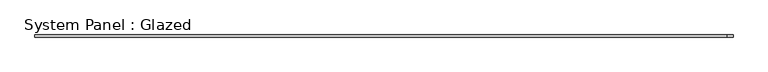
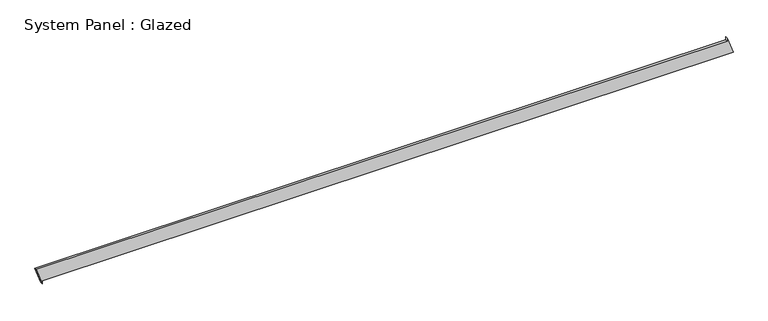
"""IFC4 building model written with IfcOpenShell, lengths in millimetres: plate geometry, System Panel : Glazed."""

from ifc_helpers import new_model, si_unit, frame, origin, place, context, project, spatial, polyline, outline, extrude, source, transform, mapped, element, save


def system_panel_glazed_c66885b6(model_context):
    return source(origin(), model_context, "Body", "SweptSolid", [
        extrude(outline(polyline([(0.0, -3956.9172633), (35.3553391, -3956.9172633), (35.3553391, 4026.9889068), (234.167386, 3956.9192133), (198.8120469, 3956.919217), (198.8112207, -4026.9889068), (0.0, -3956.9172633)])), frame((0.0, -49.5, 0.0), z_axis=(0.0, 1.0, 0.0), x_axis=(0.0, 0.0, 1.0)), (0.0, 0.0, 1.0), 25.0),
    ])


if __name__ == "__main__":
    model = new_model("IFC4")
    model_context = context("Model", 3, world=origin())
    ifc_project = project(units=[si_unit("LENGTHUNIT", "METRE", prefix="MILLI")], contexts=[model_context])
    site = spatial("IfcSite", under=ifc_project)
    building = spatial("IfcBuilding", under=site)
    placement = place(None, origin())
    system_panel_glazed_shape = system_panel_glazed_c66885b6(model_context)
    element("IfcPlate", 1, ObjectType="System Panel : Glazed", at=placement, inside=building, context=model_context, shape_type="MappedRepresentation", body=[
        mapped(system_panel_glazed_shape, transform((0.0, 0.0, 0.0), x_axis=(1.0, 0.0, 0.0), y_axis=(0.0, 1.0, 0.0), z_axis=(0.0, 0.0, 1.0))),
    ])
    save(model, "model.ifc")

# Revit data of these elements
# Element 1 (IfcPlate, "System Panel : Glazed")
#   Materials on its faces: "Glass"
# Materials
#   "Glass": class "Glass", colour RGB 218 227 224, transparency 0.85, Description = "Soda Lime Glass", Cost = 0
